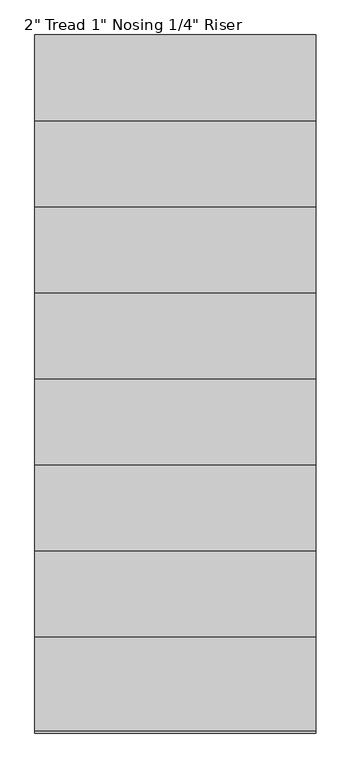
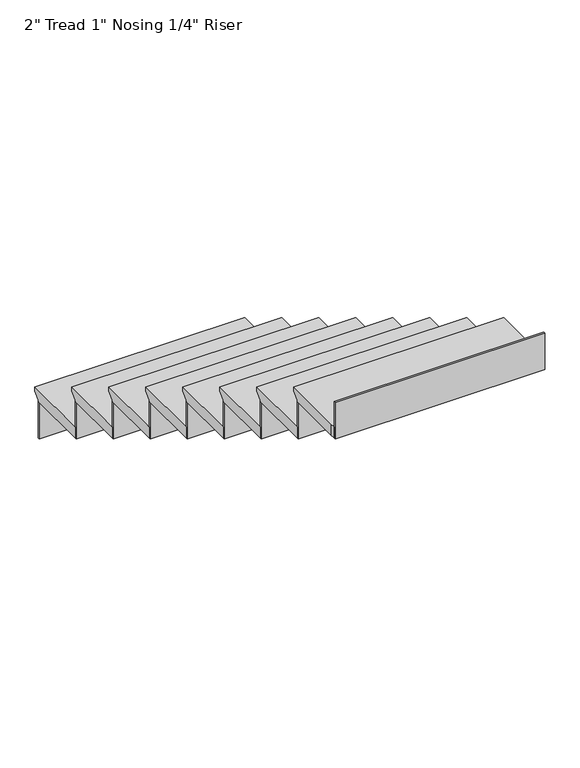
"""IFC4 building model written with IfcOpenShell, lengths in millimetres: stair flight geometry."""

from ifc_helpers import new_model, si_unit, origin, place, context, project, spatial, faceted_brep, source, transform, mapped, element, save


def stair_flight_f54f5c46(model_context):
    return source(origin(), model_context, "Body", "Brep", [
        faceted_brep([(16995.9123343, 17121.2483822, 1693.3333333), (16081.5123343, 17121.2483822, 1693.3333333), (16081.5123343, 16816.4483822, 1693.3333333), (16995.9123343, 16816.4483822, 1693.3333333), (16995.9123343, 17095.8483822, 1642.5333333), (16995.9123343, 16816.4483822, 1642.5333333), (16081.5123343, 16816.4483822, 1642.5333333), (16081.5123343, 17095.8483822, 1642.5333333), (16995.9123343, 17095.8483822, 1648.8833333), (16995.9123343, 17121.2483822, 1674.2833333), (16081.5123343, 17095.8483822, 1648.8833333), (16081.5123343, 17121.2483822, 1674.2833333)], [[[0, 1, 2, 3]], [[4, 5, 6, 7]], [[0, 3, 5, 4, 8, 9]], [[4, 7, 10, 8]], [[2, 1, 11, 10, 7, 6]], [[3, 2, 6, 5]], [[11, 1, 0, 9]], [[10, 11, 9, 8]]]),
        faceted_brep([(16081.5123343, 17095.8483822, 1642.5333333), (16081.5123343, 17095.8483822, 1473.2), (16081.5123343, 17089.4983822, 1473.2), (16081.5123343, 17089.4983822, 1642.5333333), (16995.9123343, 17095.8483822, 1642.5333333), (16995.9123343, 17089.4983822, 1642.5333333), (16995.9123343, 17089.4983822, 1473.2), (16995.9123343, 17095.8483822, 1473.2)], [[[0, 1, 2, 3]], [[4, 5, 6, 7]], [[1, 0, 4, 7]], [[2, 1, 7, 6]], [[3, 2, 6, 5]], [[0, 3, 5, 4]]]),
        faceted_brep([(16995.9123343, 16841.8483822, 1862.6666667), (16081.5123343, 16841.8483822, 1862.6666667), (16081.5123343, 16537.0483822, 1862.6666667), (16995.9123343, 16537.0483822, 1862.6666667), (16995.9123343, 16816.4483822, 1811.8666667), (16995.9123343, 16537.0483822, 1811.8666667), (16081.5123343, 16537.0483822, 1811.8666667), (16081.5123343, 16816.4483822, 1811.8666667), (16995.9123343, 16816.4483822, 1818.2166667), (16995.9123343, 16841.8483822, 1843.6166667), (16081.5123343, 16816.4483822, 1818.2166667), (16081.5123343, 16841.8483822, 1843.6166667)], [[[0, 1, 2, 3]], [[4, 5, 6, 7]], [[0, 3, 5, 4, 8, 9]], [[4, 7, 10, 8]], [[2, 1, 11, 10, 7, 6]], [[3, 2, 6, 5]], [[11, 1, 0, 9]], [[10, 11, 9, 8]]]),
        faceted_brep([(16081.5123343, 16816.4483822, 1811.8666667), (16081.5123343, 16816.4483822, 1642.5333333), (16081.5123343, 16810.0983822, 1642.5333333), (16081.5123343, 16810.0983822, 1811.8666667), (16995.9123343, 16816.4483822, 1811.8666667), (16995.9123343, 16810.0983822, 1811.8666667), (16995.9123343, 16810.0983822, 1642.5333333), (16995.9123343, 16816.4483822, 1642.5333333)], [[[0, 1, 2, 3]], [[4, 5, 6, 7]], [[1, 0, 4, 7]], [[2, 1, 7, 6]], [[3, 2, 6, 5]], [[0, 3, 5, 4]]]),
        faceted_brep([(16995.9123343, 16562.4483822, 2032.0), (16081.5123343, 16562.4483822, 2032.0), (16081.5123343, 16257.6483822, 2032.0), (16995.9123343, 16257.6483822, 2032.0), (16995.9123343, 16537.0483822, 1981.2), (16995.9123343, 16257.6483822, 1981.2), (16081.5123343, 16257.6483822, 1981.2), (16081.5123343, 16537.0483822, 1981.2), (16995.9123343, 16537.0483822, 1987.55), (16995.9123343, 16562.4483822, 2012.95), (16081.5123343, 16537.0483822, 1987.55), (16081.5123343, 16562.4483822, 2012.95)], [[[0, 1, 2, 3]], [[4, 5, 6, 7]], [[0, 3, 5, 4, 8, 9]], [[4, 7, 10, 8]], [[2, 1, 11, 10, 7, 6]], [[3, 2, 6, 5]], [[11, 1, 0, 9]], [[10, 11, 9, 8]]]),
        faceted_brep([(16081.5123343, 16537.0483822, 1981.2), (16081.5123343, 16537.0483822, 1811.8666667), (16081.5123343, 16530.6983822, 1811.8666667), (16081.5123343, 16530.6983822, 1981.2), (16995.9123343, 16537.0483822, 1981.2), (16995.9123343, 16530.6983822, 1981.2), (16995.9123343, 16530.6983822, 1811.8666667), (16995.9123343, 16537.0483822, 1811.8666667)], [[[0, 1, 2, 3]], [[4, 5, 6, 7]], [[1, 0, 4, 7]], [[2, 1, 7, 6]], [[3, 2, 6, 5]], [[0, 3, 5, 4]]]),
        faceted_brep([(16995.9123343, 16283.0483822, 2201.3333333), (16081.5123343, 16283.0483822, 2201.3333333), (16081.5123343, 15978.2483822, 2201.3333333), (16995.9123343, 15978.2483822, 2201.3333333), (16995.9123343, 16257.6483822, 2150.5333333), (16995.9123343, 15978.2483822, 2150.5333333), (16081.5123343, 15978.2483822, 2150.5333333), (16081.5123343, 16257.6483822, 2150.5333333), (16995.9123343, 16257.6483822, 2156.8833333), (16995.9123343, 16283.0483822, 2182.2833333), (16081.5123343, 16257.6483822, 2156.8833333), (16081.5123343, 16283.0483822, 2182.2833333)], [[[0, 1, 2, 3]], [[4, 5, 6, 7]], [[0, 3, 5, 4, 8, 9]], [[4, 7, 10, 8]], [[2, 1, 11, 10, 7, 6]], [[3, 2, 6, 5]], [[11, 1, 0, 9]], [[10, 11, 9, 8]]]),
        faceted_brep([(16081.5123343, 16257.6483822, 2150.5333333), (16081.5123343, 16257.6483822, 1981.2), (16081.5123343, 16251.2983822, 1981.2), (16081.5123343, 16251.2983822, 2150.5333333), (16995.9123343, 16257.6483822, 2150.5333333), (16995.9123343, 16251.2983822, 2150.5333333), (16995.9123343, 16251.2983822, 1981.2), (16995.9123343, 16257.6483822, 1981.2)], [[[0, 1, 2, 3]], [[4, 5, 6, 7]], [[1, 0, 4, 7]], [[2, 1, 7, 6]], [[3, 2, 6, 5]], [[0, 3, 5, 4]]]),
        faceted_brep([(16995.9123343, 16003.6483822, 2370.6666667), (16081.5123343, 16003.6483822, 2370.6666667), (16081.5123343, 15698.8483822, 2370.6666667), (16995.9123343, 15698.8483822, 2370.6666667), (16995.9123343, 15978.2483822, 2319.8666667), (16995.9123343, 15698.8483822, 2319.8666667), (16081.5123343, 15698.8483822, 2319.8666667), (16081.5123343, 15978.2483822, 2319.8666667), (16995.9123343, 15978.2483822, 2326.2166667), (16995.9123343, 16003.6483822, 2351.6166667), (16081.5123343, 15978.2483822, 2326.2166667), (16081.5123343, 16003.6483822, 2351.6166667)], [[[0, 1, 2, 3]], [[4, 5, 6, 7]], [[0, 3, 5, 4, 8, 9]], [[4, 7, 10, 8]], [[2, 1, 11, 10, 7, 6]], [[3, 2, 6, 5]], [[11, 1, 0, 9]], [[10, 11, 9, 8]]]),
        faceted_brep([(16081.5123343, 15978.2483822, 2319.8666667), (16081.5123343, 15978.2483822, 2150.5333333), (16081.5123343, 15971.8983822, 2150.5333333), (16081.5123343, 15971.8983822, 2319.8666667), (16995.9123343, 15978.2483822, 2319.8666667), (16995.9123343, 15971.8983822, 2319.8666667), (16995.9123343, 15971.8983822, 2150.5333333), (16995.9123343, 15978.2483822, 2150.5333333)], [[[0, 1, 2, 3]], [[4, 5, 6, 7]], [[1, 0, 4, 7]], [[2, 1, 7, 6]], [[3, 2, 6, 5]], [[0, 3, 5, 4]]]),
        faceted_brep([(16995.9123343, 15724.2483822, 2540.0), (16081.5123343, 15724.2483822, 2540.0), (16081.5123343, 15419.4483822, 2540.0), (16995.9123343, 15419.4483822, 2540.0), (16995.9123343, 15698.8483822, 2489.2), (16995.9123343, 15419.4483822, 2489.2), (16081.5123343, 15419.4483822, 2489.2), (16081.5123343, 15698.8483822, 2489.2), (16995.9123343, 15698.8483822, 2495.55), (16995.9123343, 15724.2483822, 2520.95), (16081.5123343, 15698.8483822, 2495.55), (16081.5123343, 15724.2483822, 2520.95)], [[[0, 1, 2, 3]], [[4, 5, 6, 7]], [[0, 3, 5, 4, 8, 9]], [[4, 7, 10, 8]], [[2, 1, 11, 10, 7, 6]], [[3, 2, 6, 5]], [[11, 1, 0, 9]], [[10, 11, 9, 8]]]),
        faceted_brep([(16081.5123343, 15698.8483822, 2489.2), (16081.5123343, 15698.8483822, 2319.8666667), (16081.5123343, 15692.4983822, 2319.8666667), (16081.5123343, 15692.4983822, 2489.2), (16995.9123343, 15698.8483822, 2489.2), (16995.9123343, 15692.4983822, 2489.2), (16995.9123343, 15692.4983822, 2319.8666667), (16995.9123343, 15698.8483822, 2319.8666667)], [[[0, 1, 2, 3]], [[4, 5, 6, 7]], [[1, 0, 4, 7]], [[2, 1, 7, 6]], [[3, 2, 6, 5]], [[0, 3, 5, 4]]]),
        faceted_brep([(16995.9123343, 15444.8483822, 2709.3333333), (16081.5123343, 15444.8483822, 2709.3333333), (16081.5123343, 15140.0483822, 2709.3333333), (16995.9123343, 15140.0483822, 2709.3333333), (16995.9123343, 15419.4483822, 2658.5333333), (16995.9123343, 15140.0483822, 2658.5333333), (16081.5123343, 15140.0483822, 2658.5333333), (16081.5123343, 15419.4483822, 2658.5333333), (16995.9123343, 15419.4483822, 2664.8833333), (16995.9123343, 15444.8483822, 2690.2833333), (16081.5123343, 15419.4483822, 2664.8833333), (16081.5123343, 15444.8483822, 2690.2833333)], [[[0, 1, 2, 3]], [[4, 5, 6, 7]], [[0, 3, 5, 4, 8, 9]], [[4, 7, 10, 8]], [[2, 1, 11, 10, 7, 6]], [[3, 2, 6, 5]], [[11, 1, 0, 9]], [[10, 11, 9, 8]]]),
        faceted_brep([(16081.5123343, 15419.4483822, 2658.5333333), (16081.5123343, 15419.4483822, 2489.2), (16081.5123343, 15413.0983822, 2489.2), (16081.5123343, 15413.0983822, 2658.5333333), (16995.9123343, 15419.4483822, 2658.5333333), (16995.9123343, 15413.0983822, 2658.5333333), (16995.9123343, 15413.0983822, 2489.2), (16995.9123343, 15419.4483822, 2489.2)], [[[0, 1, 2, 3]], [[4, 5, 6, 7]], [[1, 0, 4, 7]], [[2, 1, 7, 6]], [[3, 2, 6, 5]], [[0, 3, 5, 4]]]),
        faceted_brep([(16995.9123343, 14860.6483822, 2878.6666667), (16995.9123343, 14886.0483822, 2878.6666667), (16995.9123343, 15165.4483822, 2878.6666667), (16081.5123343, 15165.4483822, 2878.6666667), (16081.5123343, 14886.0483822, 2878.6666667), (16081.5123343, 14860.6483822, 2878.6666667), (16995.9123343, 14886.0483822, 2827.8666667), (16995.9123343, 14860.6483822, 2827.8666667), (16081.5123343, 14860.6483822, 2827.8666667), (16081.5123343, 14886.0483822, 2827.8666667), (16081.5123343, 15140.0483822, 2827.8666667), (16995.9123343, 15140.0483822, 2827.8666667), (16081.5123343, 15140.0483822, 2834.2166667), (16995.9123343, 15140.0483822, 2834.2166667), (16081.5123343, 15165.4483822, 2859.6166667), (16995.9123343, 15165.4483822, 2859.6166667)], [[[0, 1, 2, 3, 4, 5]], [[6, 7, 8, 9, 10, 11]], [[1, 0, 7, 6]], [[11, 10, 12, 13]], [[4, 3, 14, 12, 10, 9]], [[0, 5, 8, 7]], [[14, 3, 2, 15]], [[12, 14, 15, 13]], [[2, 1, 6, 11, 13, 15]], [[5, 4, 9, 8]]]),
        faceted_brep([(16081.5123343, 15140.0483822, 2827.8666667), (16081.5123343, 15140.0483822, 2658.5333333), (16081.5123343, 15133.6983822, 2658.5333333), (16081.5123343, 15133.6983822, 2827.8666667), (16995.9123343, 15140.0483822, 2827.8666667), (16995.9123343, 15133.6983822, 2827.8666667), (16995.9123343, 15133.6983822, 2658.5333333), (16995.9123343, 15140.0483822, 2658.5333333)], [[[0, 1, 2, 3]], [[4, 5, 6, 7]], [[1, 0, 4, 7]], [[2, 1, 7, 6]], [[3, 2, 6, 5]], [[0, 3, 5, 4]]]),
        faceted_brep([(16081.5123343, 14860.6483822, 2997.2), (16081.5123343, 14860.6483822, 2827.8666667), (16081.5123343, 14854.2983822, 2827.8666667), (16081.5123343, 14854.2983822, 2997.2), (16995.9123343, 14860.6483822, 2997.2), (16995.9123343, 14854.2983822, 2997.2), (16995.9123343, 14854.2983822, 2827.8666667), (16995.9123343, 14860.6483822, 2827.8666667)], [[[0, 1, 2, 3]], [[4, 5, 6, 7]], [[1, 0, 4, 7]], [[2, 1, 7, 6]], [[3, 2, 6, 5]], [[0, 3, 5, 4]]]),
    ])


if __name__ == "__main__":
    model = new_model("IFC4")
    model_context = context("Model", 3, world=origin())
    ifc_project = project(units=[si_unit("LENGTHUNIT", "METRE", prefix="MILLI")], contexts=[model_context])
    site = spatial("IfcSite", under=ifc_project)
    building = spatial("IfcBuilding", under=site)
    placement = place(None, origin())
    stair_flight_shape = stair_flight_f54f5c46(model_context)
    element("IfcStairFlight", 1, ObjectType="2\" Tread 1\" Nosing 1/4\" Riser", at=placement, inside=building, context=model_context, shape_type="MappedRepresentation", body=[
        mapped(stair_flight_shape, transform((0.0, 0.0, 0.0), x_axis=(1.0, 0.0, 0.0), y_axis=(0.0, 1.0, 0.0), z_axis=(0.0, 0.0, 1.0))),
    ])
    save(model, "model.ifc")

# Revit data of these elements
# Element 1 (IfcStairFlight, "2\" Tread 1\" Nosing 1/4\" Riser")
#   Materials on its faces: "Oak Flooring"
# Materials
#   "Oak Flooring": class "Wood", colour RGB 216 169 114, transparency 0, Description = "Quercus Rubra", Cost = 0
